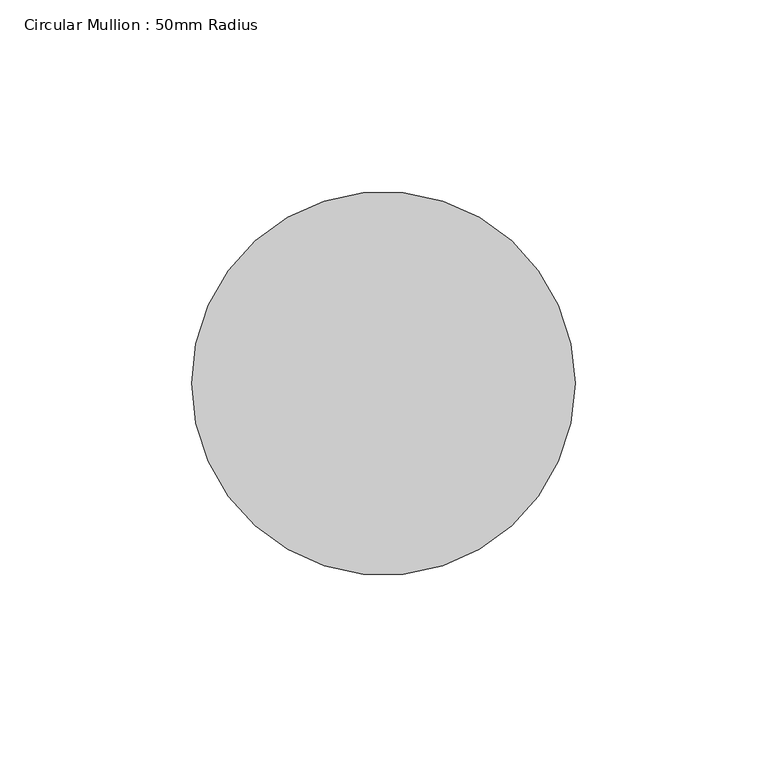
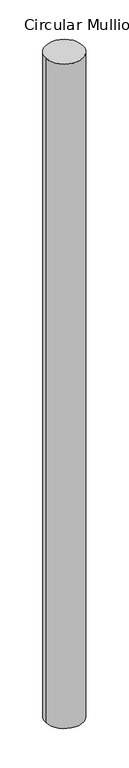
"""IFC4 building model written with IfcOpenShell, lengths in millimetres: member geometry, Circular Mullion : 50mm Radius."""

from ifc_helpers import new_model, si_unit, point, frame, origin, origin_2d, place, context, project, spatial, circle_curve, trimmed, segment, composite_curve, outline, extrude, source, transform, mapped, element, save


def circular_mullion_50mm_radius_d8d511d0(model_context):
    return source(origin(), model_context, "Body", "SweptSolid", [
        extrude(outline(composite_curve([segment(trimmed(circle_curve(origin_2d(), 50.0), [point((50.0, 0.0))], [point((-50.0, 0.0))], False, "CARTESIAN"), True, "CONTINUOUS"), segment(trimmed(circle_curve(origin_2d(), 50.0), [point((-50.0, 0.0))], [point((50.0, 0.0))], False, "CARTESIAN"), True, "CONTINUOUS")], self_intersect=False)), frame((0.0, 0.0, -1883.8169373), z_axis=(0.0, 0.0, 1.0), x_axis=(1.0, 0.0, 0.0)), (0.0, 0.0, 1.0), 1883.8169373),
    ])


if __name__ == "__main__":
    model = new_model("IFC4")
    model_context = context("Model", 3, world=origin())
    ifc_project = project(units=[si_unit("LENGTHUNIT", "METRE", prefix="MILLI")], contexts=[model_context])
    site = spatial("IfcSite", under=ifc_project)
    building = spatial("IfcBuilding", under=site)
    placement = place(None, origin())
    circular_mullion_50mm_radius_shape = circular_mullion_50mm_radius_d8d511d0(model_context)
    element("IfcMember", 1, ObjectType="Circular Mullion : 50mm Radius", at=placement, inside=building, context=model_context, shape_type="MappedRepresentation", body=[
        mapped(circular_mullion_50mm_radius_shape, transform((0.0, 0.0, 0.0), x_axis=(1.0, 0.0, 0.0), y_axis=(0.0, 1.0, 0.0), z_axis=(0.0, 0.0, 1.0))),
    ])
    save(model, "model.ifc")

# Revit data of these elements
# Type "Circular Mullion : 50mm Radius"
#   built-in parameter 1007350 = 0.164042 (stored number, unit not read)
# Element 1 (IfcMember, "Circular Mullion : 50mm Radius")
#   Materials on its faces: "Aluminium"
# Materials
#   "Aluminium": class "Metal", colour RGB 247 247 247, transparency 0, Description = "Aluminium 6061", Cost = 0
